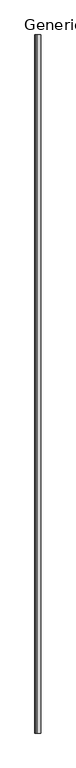
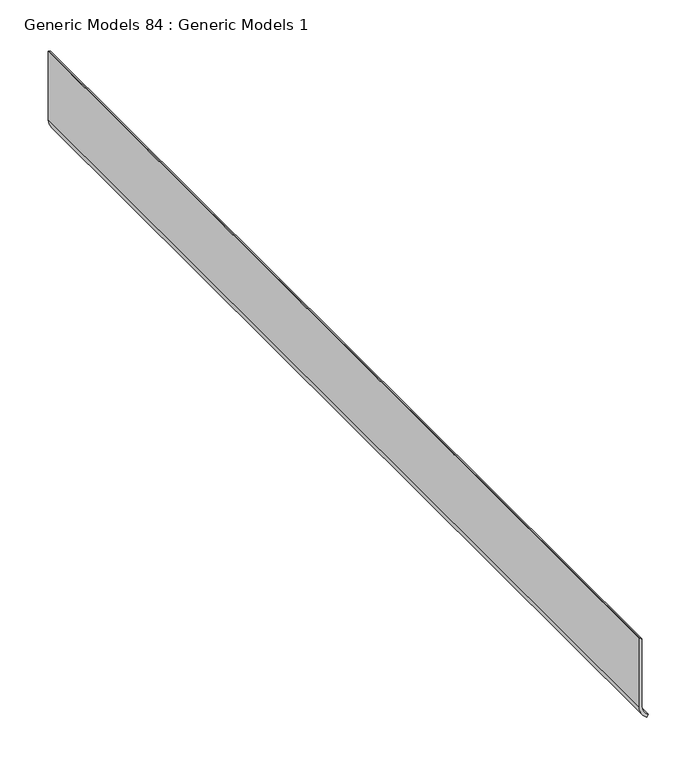
"""IFC4 building model written with IfcOpenShell, lengths in millimetres: proxy geometry, Generic Models 84 : Generic Models 1."""

from ifc_helpers import new_model, si_unit, point, frame, frame_2d, origin, place, context, project, spatial, polyline, circle_curve, trimmed, segment, composite_curve, outline, extrude, source, transform, mapped, element, save


def generic_models_84_generic_models_1_ca595b11(model_context):
    return source(origin(), model_context, "Body", "SweptSolid", [
        extrude(outline(composite_curve([segment(polyline([(-2048.8233876, 49818.1931639), (-2134.9737569, 49818.1931639)]), True, "CONTINUOUS"), segment(trimmed(circle_curve(frame_2d((-2134.9737569, 49836.0328607)), 17.8396968), [point((-2134.9737569, 49818.1931639))], [point((-2150.4233876, 49827.1130123))], False, "CARTESIAN"), True, "CONTINUOUS"), segment(polyline([(-2150.4233876, 49827.1130123), (-2147.6737569, 49828.7005123)]), True, "CONTINUOUS"), segment(trimmed(circle_curve(frame_2d((-2134.9737569, 49836.0328607)), 14.6646968), [point((-2147.6737569, 49828.7005123))], [point((-2134.9737569, 49821.3681639))], True, "CARTESIAN"), True, "CONTINUOUS"), segment(polyline([(-2134.9737569, 49821.3681639), (-2050.9101894, 49821.3681639)]), True, "CONTINUOUS"), segment(trimmed(circle_curve(frame_2d((-2050.9101894, 49819.2813621)), 2.0868018), [point((-2050.9101894, 49821.3681639))], [point((-2048.8233876, 49819.2813621))], False, "CARTESIAN"), True, "CONTINUOUS"), segment(polyline([(-2048.8233876, 49819.2813621), (-2048.8233876, 49818.1931639)]), True, "CONTINUOUS")], self_intersect=False)), frame((0.0, 0.0, 0.0), z_axis=(0.0, 1.0, 0.0), x_axis=(0.0, 0.0, 1.0)), (0.0, 0.0, 1.0), 1219.2),
    ])


if __name__ == "__main__":
    model = new_model("IFC4")
    model_context = context("Model", 3, world=origin())
    ifc_project = project(units=[si_unit("LENGTHUNIT", "METRE", prefix="MILLI")], contexts=[model_context])
    site = spatial("IfcSite", under=ifc_project)
    building = spatial("IfcBuilding", under=site)
    placement = place(None, origin())
    generic_models_84_generic_models_1_shape = generic_models_84_generic_models_1_ca595b11(model_context)
    element("IfcBuildingElementProxy", 1, Name="Generic Models 84 : Generic Models 1", ObjectType="Generic Models 84 : Generic Models 1", at=placement, inside=building, context=model_context, shape_type="MappedRepresentation", body=[
        mapped(generic_models_84_generic_models_1_shape, transform((0.0, 0.0, 0.0), x_axis=(1.0, 0.0, 0.0), y_axis=(0.0, 1.0, 0.0), z_axis=(0.0, 0.0, 1.0))),
    ])
    save(model, "model.ifc")

# Revit data of these elements
# Element 1 (IfcBuildingElementProxy, "Generic Models 84 : Generic Models 1")
#   Materials on its faces: "BASE T.B.D."
# Materials
#   "BASE T.B.D.": class "Generic", colour RGB 120 120 120, transparency 0, Cost = 0
